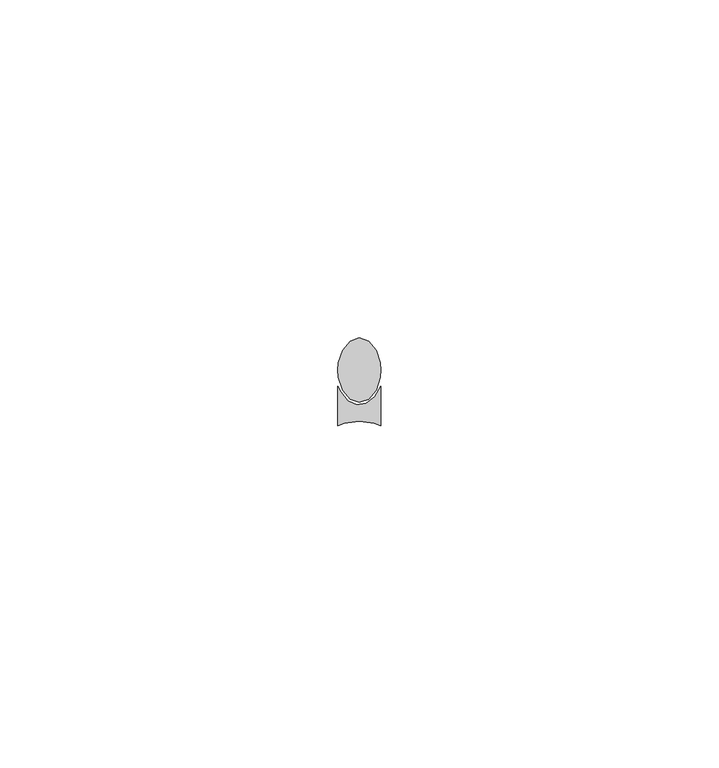
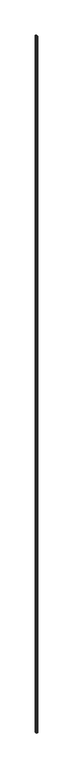
"""IFC4 building model written with IfcOpenShell, lengths in millimetres: proxy geometry, Generic Models 11:Generic Models 1:306267:Generic Models 1:306267 : Generic Models 11:Generic Models 1:306267:300405:Generic Models 1:306267:Generic Models 1:306267 : Generic Models 11:Generic Models 1:306267:300405 : Generic Models 11:Generic Models 1:306267:Generic Models 1:306267 : Generic Models 11:Generic Models 1:306267:300405:1 : Generic Models 11:Generic Models 1:306267:Generic Models 1:306267 : Generic Models 11:Generic Models 1:306267:300405:Generic Models 1:306267:Generic Models 1:306267 : Generic Models 11:Generic Models 1:306267:300405 : Generic Models 11:Generic Models 1:306267:Generic Models 1:306267 : Generic Models 11:Generic Models 1:306267:300405:300182."""

from ifc_helpers import new_model, si_unit, origin, origin_with_axes, place, context, project, spatial, polyline, outline, extrude, source, transform, mapped, element, save


def generic_models_d83d58e7(model_context):
    return source(origin(), model_context, "Body", "SweptSolid", [
        extrude(outline(polyline([(593733.5341431, -579092.0005286), (593732.429409, -579090.6790346), (593731.8163278, -579088.7694203), (593731.7367239, -579087.7096644), (593731.8163278, -579086.6499084), (593732.429409, -579084.7402942), (593733.5341431, -579083.4188002), (593734.9117239, -579082.9471644), (593736.2893048, -579083.4188002), (593737.3940389, -579084.7402942), (593738.0071201, -579086.6499084), (593738.0867239, -579087.7096644), (593738.0071201, -579088.7694203), (593737.3940389, -579090.6790346), (593736.2893048, -579092.0005286), (593734.9117239, -579092.4721644), (593733.5341431, -579092.0005286)])), origin_with_axes(), (0.0, 0.0, 1.0), 3695.7),
        extrude(outline(polyline([(593737.1209607, -579095.5639755), (593734.9117239, -579095.2502894), (593732.7024872, -579095.5639755), (593731.7367239, -579095.9413841), (593731.7367239, -579090.073292), (593732.1230415, -579090.9335729), (593733.206527, -579092.2431481), (593734.5567747, -579092.8435016), (593735.962551, -579092.6407137), (593737.2039351, -579091.6665087), (593738.0867239, -579090.073292), (593738.0867239, -579095.9413841), (593737.1209607, -579095.5639755)])), origin_with_axes(), (0.0, 0.0, 1.0), 3695.7),
    ])


if __name__ == "__main__":
    model = new_model("IFC4")
    model_context = context("Model", 3, world=origin())
    ifc_project = project(units=[si_unit("LENGTHUNIT", "METRE", prefix="MILLI")], contexts=[model_context])
    site = spatial("IfcSite", under=ifc_project)
    building = spatial("IfcBuilding", under=site)
    placement = place(None, origin())
    generic_models_shape = generic_models_d83d58e7(model_context)
    element("IfcBuildingElementProxy", 1, Name="Generic Models 11:Generic Models 1:306267:Generic Models 1:306267 : Generic Models 11:Generic Models 1:306267:300405:Generic Models 1:306267:Generic Models 1:306267 : Generic Models 11:Generic Models 1:306267:300405 : Generic Models 11:Generic Models 1:306267:Generic Models 1:306267 : Generic Models 11:Generic Models 1:306267:300405:1 : Generic Models 11:Generic Models 1:306267:Generic Models 1:306267 : Generic Models 11:Generic Models 1:306267:300405:Generic Models 1:306267:Generic Models 1:306267 : Generic Models 11:Generic Models 1:306267:300405 : Generic Models 11:Generic Models 1:306267:Generic Models 1:306267 : Generic Models 11:Generic Models 1:306267:300405:300182", ObjectType="Generic Models 11:Generic Models 1:306267:Generic Models 1:306267 : Generic Models 11:Generic Models 1:306267:300405:Generic Models 1:306267:Generic Models 1:306267 : Generic Models 11:Generic Models 1:306267:300405 : Generic Models 11:Generic Models 1:306267:Generic Models 1:306267 : Generic Models 11:Generic Models 1:306267:300405:1 : Generic Models 11:Generic Models 1:306267:Generic Models 1:306267 : Generic Models 11:Generic Models 1:306267:300405:Generic Models 1:306267:Generic Models 1:306267 : Generic Models 11:Generic Models 1:306267:300405 : Generic Models 11:Generic Models 1:306267:Generic Models 1:306267 : Generic Models 11:Generic Models 1:306267:300405:300182", at=placement, inside=building, context=model_context, shape_type="MappedRepresentation", body=[
        mapped(generic_models_shape, transform((0.0, 0.0, 0.0), x_axis=(1.0, 0.0, 0.0), y_axis=(0.0, 1.0, 0.0), z_axis=(0.0, 0.0, 1.0))),
    ])
    save(model, "model.ifc")

# Revit data of these elements
# Type "Generic Models 11:Generic Models 1:306267:Generic Models 1:306267 : Generic Models 11:Generic Models 1:306267:300405:Generic Models 1:306267:Generic Models 1:306267 : Generic Models 11:Generic Models 1:306267:300405 : Generic Models 11:Generic Models 1:306267:Generic Models 1:306267 : Generic Models 11:Generic Models 1:306267:300405:1 : Generic Models 11:Generic Models 1:306267:Generic Models 1:306267 : Generic Models 11:Generic Models 1:306267:300405:Generic Models 1:306267:Generic Models 1:306267 : Generic Models 11:Generic Models 1:306267:300405 : Generic Models 11:Generic Models 1:306267:Generic Models 1:306267 : Generic Models 11:Generic Models 1:306267:300405:300182"
#   NameOverride = "Generic Models 11:Generic Models 1:306267:Generic Models 1:306267 : Generic Models 11:Generic Models 1:306267:300405:Generic Models 1:306267:Generic Models 1:306267 : Generic Models 11:Generic Models 1:306267:300405 : Generic Models 11:Generic Models 1:306267:Generic Models 1:306267 : Generic Models 11:Generic Models 1:306267:300405:300182"
#   ObjectTypeOverride = "Generic Models 1:306267:Generic Models 1:306267 : Generic Models 11:Generic Models 1:306267:300405 : Generic Models 11:Generic Models 1:306267:Generic Models 1:306267 : Generic Models 11:Generic Models 1:306267:300405"
#   Reference = "Generic Models 1"
#   Tag = "300182"
# Element 1 (IfcBuildingElementProxy, "Generic Models 11:Generic Models 1:306267:Generic Models 1:306267 : Generic Models 11:Generic Models 1:306267:300405:Generic Models 1:306267:Generic Models 1:306267 : Generic Models 11:Generic Models 1:306267:300405 : Generic Models 11:Generic Models 1:306267:Generic Models 1:306267 : Generic Models 11:Generic Models 1:306267:300405:1 : Generic Models 11:Generic Models 1:306267:Generic Models 1:306267 : Generic Models 11:Generic Models 1:306267:300405:Generic Models 1:306267:Generic Models 1:306267 : Generic Models 11:Generic Models 1:306267:300405 : Generic Models 11:Generic Models 1:306267:Generic Models 1:306267 : Generic Models 11:Generic Models 1:306267:300405:300182")
#   Materials on its faces: "SEALANT & BACKER ROD"
# Materials
#   "SEALANT & BACKER ROD": class "Unassigned", colour RGB 120 120 120, transparency 0, Cost = 0
